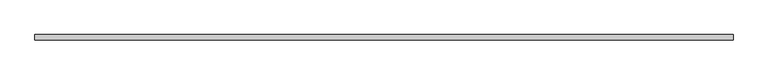
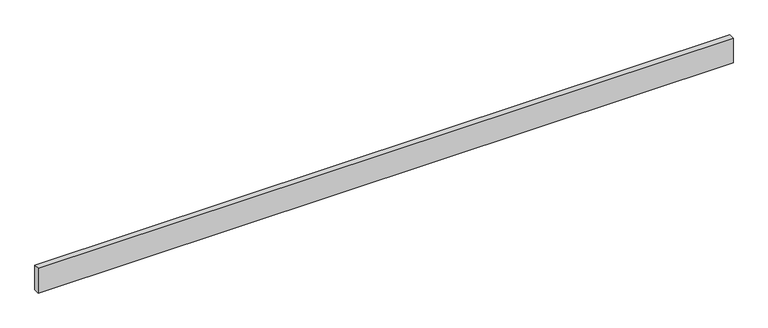
"""IFC4 building model written with IfcOpenShell, lengths in millimetres: proxy geometry, Generic Models 7:Generic Models 1:2:Generic Models 1:2 : Generic Models 7:Generic Models 1:337419:7 : Generic Models 7:Generic Models 1:2:Generic Models 1:2 : Generic Models 7:Generic Models 1:337419:306751."""

from ifc_helpers import new_model, si_unit, frame, origin, place, context, project, spatial, polyline, outline, extrude, source, transform, mapped, element, save


def generic_models_01d25e4b(model_context):
    return source(origin(), model_context, "Body", "SweptSolid", [
        extrude(outline(polyline([(596182.8367239, -579030.8538841), (596182.8367239, -579068.9538841), (591306.0367239, -579068.9538841), (591306.0367239, -579030.8538841), (596182.8367239, -579030.8538841)])), frame((0.0, 0.0, 3721.8937499), z_axis=(0.0, 0.0, 1.0), x_axis=(1.0, 0.0, 0.0)), (0.0, 0.0, 1.0), 184.15),
    ])


if __name__ == "__main__":
    model = new_model("IFC4")
    model_context = context("Model", 3, world=origin())
    ifc_project = project(units=[si_unit("LENGTHUNIT", "METRE", prefix="MILLI")], contexts=[model_context])
    site = spatial("IfcSite", under=ifc_project)
    building = spatial("IfcBuilding", under=site)
    placement = place(None, origin())
    generic_models_shape = generic_models_01d25e4b(model_context)
    element("IfcBuildingElementProxy", 1, Name="Generic Models 7:Generic Models 1:2:Generic Models 1:2 : Generic Models 7:Generic Models 1:337419:7 : Generic Models 7:Generic Models 1:2:Generic Models 1:2 : Generic Models 7:Generic Models 1:337419:306751", ObjectType="Generic Models 7:Generic Models 1:2:Generic Models 1:2 : Generic Models 7:Generic Models 1:337419:7 : Generic Models 7:Generic Models 1:2:Generic Models 1:2 : Generic Models 7:Generic Models 1:337419:306751", at=placement, inside=building, context=model_context, shape_type="MappedRepresentation", body=[
        mapped(generic_models_shape, transform((0.0, 0.0, 0.0), x_axis=(1.0, 0.0, 0.0), y_axis=(0.0, 1.0, 0.0), z_axis=(0.0, 0.0, 1.0))),
    ])
    save(model, "model.ifc")

# Revit data of these elements
# Type "Generic Models 7:Generic Models 1:2:Generic Models 1:2 : Generic Models 7:Generic Models 1:337419:7 : Generic Models 7:Generic Models 1:2:Generic Models 1:2 : Generic Models 7:Generic Models 1:337419:306751"
#   NameOverride = "Generic Models 7:Generic Models 1:2:Generic Models 1:2 : Generic Models 7:Generic Models 1:337419:306751"
#   ObjectTypeOverride = "Generic Models 1:2 : Generic Models 7:Generic Models 1:337419"
#   Reference = "Generic Models 1"
#   Tag = "306751"
# Element 1 (IfcBuildingElementProxy, "Generic Models 7:Generic Models 1:2:Generic Models 1:2 : Generic Models 7:Generic Models 1:337419:7 : Generic Models 7:Generic Models 1:2:Generic Models 1:2 : Generic Models 7:Generic Models 1:337419:306751")
#   Materials on its faces: "BLOCKING - SIZE AS NEC."
# Materials
#   "BLOCKING - SIZE AS NEC.": class "Wood", colour RGB 144 113 62, transparency 0, Description = "Pinus Echinata", Cost = 0
